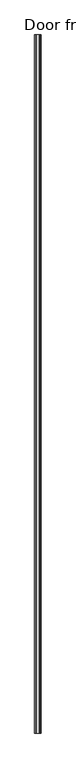
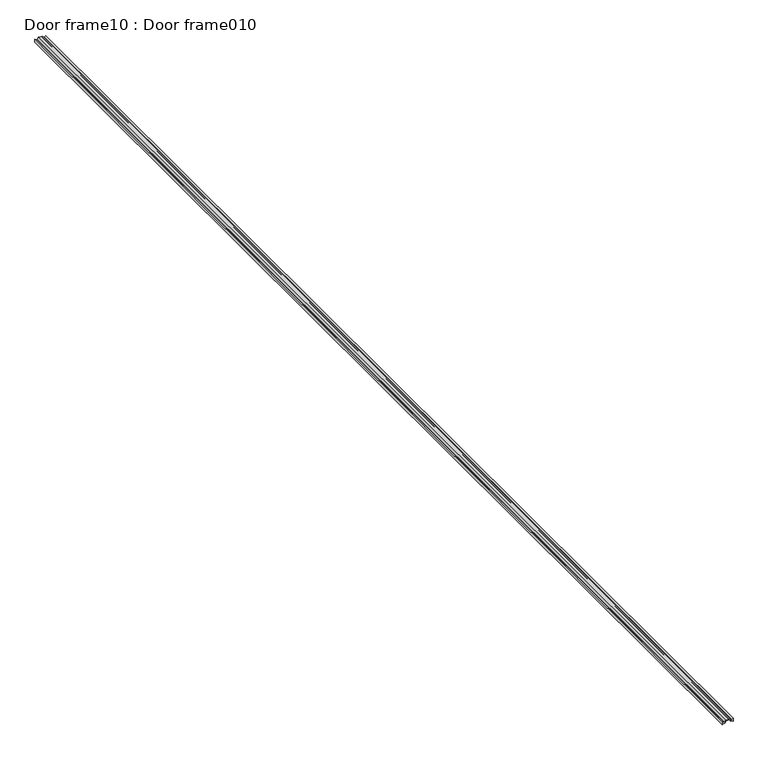
"""IFC4 building model written with IfcOpenShell, lengths in millimetres: proxy geometry, Door frame10 : Door frame010."""

import ifcopenshell
import ifcopenshell.guid

model = None  # the IFC model being written
_history = None  # IfcOwnerHistory: only IFC2X3 demands one
_inside = {}  # id of a spatial element -> (the spatial element, [elements in it])
_under = {}  # id of a project, library or spatial element -> (it, [spatial elements below it])
_declared = {}  # id of a project -> (the project, [libraries it declares])
_typed = {}  # id of a type object -> (the type object, [elements of that type])
_made_of = {}  # id of a material, layer set ... -> (it, [elements and type objects made of it])


def new_model(schema):
    """Start an empty IFC model of exactly this schema.

    Asked for "IFC4X3", IfcOpenShell would pick the latest addendum, in which some entities
    have other attributes; the version numbers below select the first issue.
    IFC2X3 requires an IfcOwnerHistory on every rooted entity: one is made here for all.
    """
    global model, _history
    if schema == "IFC4X3":
        model = ifcopenshell.file(schema_version=(4, 3, 0, 0))
    else:
        model = ifcopenshell.file(schema=schema)
    _inside.clear()
    _under.clear()
    _declared.clear()
    _typed.clear()
    _made_of.clear()
    _history = None
    if model.schema == "IFC2X3":
        org = make("IfcOrganization", Name="unknown")
        user = make(
            "IfcPersonAndOrganization",
            ThePerson=make("IfcPerson", FamilyName="unknown"),
            TheOrganization=org,
        )
        app = make(
            "IfcApplication",
            ApplicationDeveloper=org,
            Version="unknown",
            ApplicationFullName="unknown",
            ApplicationIdentifier="unknown",
        )
        _history = make(
            "IfcOwnerHistory",
            OwningUser=user,
            OwningApplication=app,
            ChangeAction="ADDED",
            CreationDate=0,
        )
    return model


def make(cls, **values):
    """One entity of the class cls with the attributes given. An attribute that is None is left unset."""
    return model.create_entity(
        cls, **{name: value for name, value in values.items() if value is not None}
    )


def rooted(cls, **values):
    """An entity with a GlobalId (a new one), such as an element, a storey or a relation."""
    return make(cls, GlobalId=ifcopenshell.guid.new(), OwnerHistory=_history, **values)


def si_unit(unit_type, name, prefix=None):
    """IfcSIUnit, for example si_unit("LENGTHUNIT", "METRE", prefix="MILLI")."""
    return make("IfcSIUnit", UnitType=unit_type, Prefix=prefix, Name=name)


def assignment(units):
    """IfcUnitAssignment: the units of a project."""
    return None if units is None else make("IfcUnitAssignment", Units=units)


def point(xyz):
    """IfcCartesianPoint."""
    return None if xyz is None else make("IfcCartesianPoint", Coordinates=xyz)


def direction(xyz):
    """IfcDirection."""
    return None if xyz is None else make("IfcDirection", DirectionRatios=xyz)


def frame(location, z_axis=None, x_axis=None):
    """IfcAxis2Placement3D, a coordinate frame: its origin and axes. An axis left out is left unset."""
    return make(
        "IfcAxis2Placement3D",
        Location=point(location),
        Axis=direction(z_axis),
        RefDirection=direction(x_axis),
    )


def origin():
    """The frame at (0, 0, 0) with its axes left unset."""
    return frame((0.0, 0.0, 0.0))


def place(relative_to, where):
    """IfcLocalPlacement: puts the frame where relative to a parent placement (None: the world)."""
    return make(
        "IfcLocalPlacement", PlacementRelTo=relative_to, RelativePlacement=where
    )


def context(
    kind, dimensions, precision=None, world=None, true_north=None, identifier=None
):
    """IfcGeometricRepresentationContext, for example the 3D "Model" context."""
    return make(
        "IfcGeometricRepresentationContext",
        ContextIdentifier=identifier,
        ContextType=kind,
        CoordinateSpaceDimension=dimensions,
        Precision=precision,
        WorldCoordinateSystem=world,
        TrueNorth=true_north,
    )


def project(units=None, contexts=None):
    """IfcProject with its units and contexts."""
    return rooted(
        "IfcProject",
        Name="project",
        RepresentationContexts=contexts,
        UnitsInContext=assignment(units),
    )


def spatial(cls, under=None, at=None, **own):
    """A site, building, storey or space (cls), placed at a placement, below another one or the project."""
    s = rooted(cls, ObjectPlacement=at, **own)
    if under is not None:
        _under.setdefault(under.id(), (under, []))[1].append(s)
    return s


def polyline(points):
    """IfcPolyline through the points."""
    return make("IfcPolyline", Points=[point(p) for p in points])


def outline(outer, holes=None, kind="AREA"):
    """IfcArbitraryClosedProfileDef: a profile drawn as a closed curve; with holes, ...WithVoids."""
    if holes is None:
        return make("IfcArbitraryClosedProfileDef", ProfileType=kind, OuterCurve=outer)
    return make(
        "IfcArbitraryProfileDefWithVoids",
        ProfileType=kind,
        OuterCurve=outer,
        InnerCurves=holes,
    )


def extrude(swept, where, along, depth):
    """IfcExtrudedAreaSolid: the profile swept, set in the frame where, extruded along a direction by depth."""
    return make(
        "IfcExtrudedAreaSolid",
        SweptArea=swept,
        Position=where,
        ExtrudedDirection=direction(along),
        Depth=depth,
    )


def shape(context_of_items, identifier, shape_type, items):
    """IfcShapeRepresentation: the items that make up one representation, for example the "Body"."""
    return make(
        "IfcShapeRepresentation",
        ContextOfItems=context_of_items,
        RepresentationIdentifier=identifier,
        RepresentationType=shape_type,
        Items=items,
    )


def source(mapping_origin, context_of_items, identifier, shape_type, items):
    """IfcRepresentationMap: a shape defined once, which mapped items show again and again."""
    return make(
        "IfcRepresentationMap",
        MappingOrigin=mapping_origin,
        MappedRepresentation=shape(context_of_items, identifier, shape_type, items),
    )


def transform(
    local_origin,
    x_axis=None,
    y_axis=None,
    z_axis=None,
    scale=None,
    scale2=None,
    scale3=None,
    uniform=True,
):
    """IfcCartesianTransformationOperator3D, or its non-uniform kind. x_axis, y_axis, z_axis: its Axis1, 2, 3."""
    if uniform:
        return make(
            "IfcCartesianTransformationOperator3D",
            Axis1=direction(x_axis),
            Axis2=direction(y_axis),
            LocalOrigin=point(local_origin),
            Scale=scale,
            Axis3=direction(z_axis),
        )
    return make(
        "IfcCartesianTransformationOperator3DnonUniform",
        Axis1=direction(x_axis),
        Axis2=direction(y_axis),
        LocalOrigin=point(local_origin),
        Scale=scale,
        Axis3=direction(z_axis),
        Scale2=scale2,
        Scale3=scale3,
    )


def mapped(mapping_source, mapping_target):
    """IfcMappedItem: shows the shape of a source again, moved by a transform."""
    return make(
        "IfcMappedItem", MappingSource=mapping_source, MappingTarget=mapping_target
    )


def made_of(thing, what):
    """Note that an element or type object is made of a material, layer set ...; save() writes the relation."""
    if what is not None:
        _made_of.setdefault(what.id(), (what, []))[1].append(thing)
    return thing


def element(
    cls,
    number,
    at=None,
    inside=None,
    cuts=None,
    type_object=None,
    material=None,
    context=None,
    identifier="Body",
    shape_type=None,
    held_by="IfcProductDefinitionShape",
    body=None,
    shapes=None,
    **own,
):
    """One element of the class cls, such as IfcWall. Its Tag is "e" and its number.

    at: its placement. inside: the storey or other place that contains it. cuts: it is an
    opening in that element (IfcRelVoidsElement). A single representation is given by context,
    identifier, shape_type and body (its items); several are given by shapes. held_by: the class
    of the entity that holds the representations. save() writes the other relations.
    """
    e = rooted(cls, Tag="e%d" % number, ObjectPlacement=at, **own)
    if body is not None:
        shapes = [shape(context, identifier, shape_type, body)]
    if shapes is not None:
        e.Representation = make(held_by, Representations=shapes)
    if inside is not None:
        _inside.setdefault(inside.id(), (inside, []))[1].append(e)
    if cuts is not None:
        rooted(
            "IfcRelVoidsElement", RelatingBuildingElement=cuts, RelatedOpeningElement=e
        )
    if type_object is not None:
        _typed.setdefault(type_object.id(), (type_object, []))[1].append(e)
    return made_of(e, material)


def aggregate(whole, parts):
    """IfcRelAggregates: a whole, such as a stair, and the parts it consists of."""
    return rooted("IfcRelAggregates", RelatingObject=whole, RelatedObjects=parts)


def save(model, path):
    """Write the relations noted so far, then the file.

    IfcRelAggregates (storeys below a building ...), IfcRelContainedInSpatialStructure (elements
    in a storey), IfcRelDefinesByType, IfcRelAssociatesMaterial and IfcRelDeclares: one each for
    every whole, place, type object, material and project.
    """
    for whole, parts in _under.values():
        aggregate(whole, parts)
    for where, things in _inside.values():
        rooted(
            "IfcRelContainedInSpatialStructure",
            RelatedElements=things,
            RelatingStructure=where,
        )
    for kind, things in _typed.values():
        rooted("IfcRelDefinesByType", RelatedObjects=things, RelatingType=kind)
    for what, things in _made_of.values():
        rooted("IfcRelAssociatesMaterial", RelatedObjects=things, RelatingMaterial=what)
    for by, libraries in _declared.values():
        rooted("IfcRelDeclares", RelatingContext=by, RelatedDefinitions=libraries)
    model.write(path)


def door_frame10_door_frame010_dc68b2cc(model_context):
    return source(origin(), model_context, "Body", "SweptSolid", [
        extrude(outline(polyline([(36662.6580816, 15538.4954576), (36662.6580816, 15540.1419606), (36665.8580816, 15542.3826247), (36665.8580816, 15547.7313685), (36662.6580816, 15549.9720326), (36662.6580816, 15551.6185356), (36661.1287449, 15554.2674246), (36665.9874184, 15554.2674246), (36664.4580816, 15551.6185356), (36664.4580816, 15550.6648984), (36667.4580816, 15548.5642757), (36667.4580816, 15541.5497174), (36664.4580816, 15539.4490948), (36664.4580816, 15538.4954576), (36666.0170308, 15535.7952784), (36661.0991325, 15535.7952784), (36662.6580816, 15538.4954576)])), frame((0.0, -1052.8906567, 0.0), z_axis=(0.0, 1.0, 0.0), x_axis=(0.0, 0.0, 1.0)), (0.0, 0.0, 1.0), 1999.85),
    ])


if __name__ == "__main__":
    model = new_model("IFC4")
    model_context = context("Model", 3, world=origin())
    ifc_project = project(units=[si_unit("LENGTHUNIT", "METRE", prefix="MILLI")], contexts=[model_context])
    site = spatial("IfcSite", under=ifc_project)
    building = spatial("IfcBuilding", under=site)
    placement = place(None, origin())
    door_frame10_door_frame010_shape = door_frame10_door_frame010_dc68b2cc(model_context)
    element("IfcBuildingElementProxy", 1, Name="Door frame10 : Door frame010", ObjectType="Door frame10 : Door frame010", at=placement, inside=building, context=model_context, shape_type="MappedRepresentation", body=[
        mapped(door_frame10_door_frame010_shape, transform((0.0, 0.0, 0.0), x_axis=(1.0, 0.0, 0.0), y_axis=(0.0, 1.0, 0.0), z_axis=(0.0, 0.0, 1.0))),
    ])
    save(model, "model.ifc")

# Revit data of these elements
# Type "Door frame10 : Door frame010"
#   NameOverride = "Door frame010"
# Element 1 (IfcBuildingElementProxy, "Door frame10 : Door frame010")
#   Materials on its faces: "FLEETWOOD SERIES T-3200 SINGLE SWING DOOR FRAME"
# Materials
#   "FLEETWOOD SERIES T-3200 SINGLE SWING DOOR FRAME": class "Unassigned", colour RGB 128 128 128, transparency 0, Cost = 0
